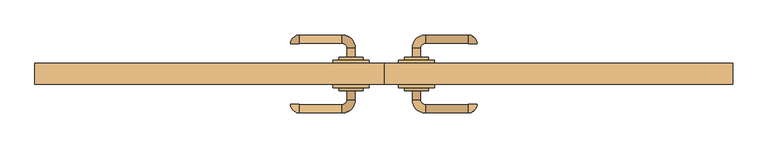
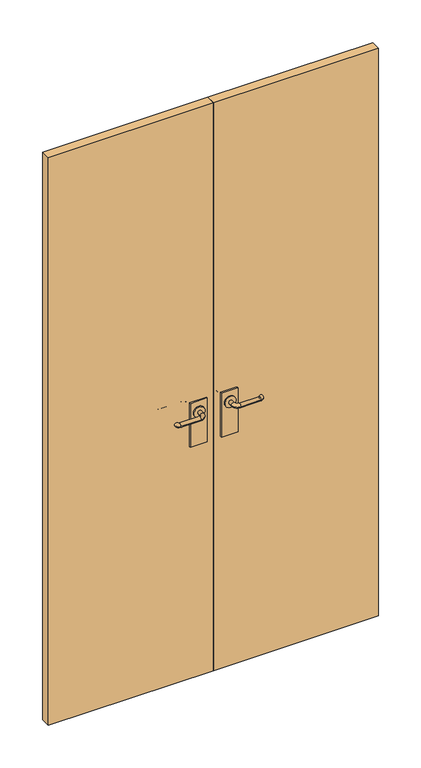
"""IFC4 building model written with IfcOpenShell, lengths in millimetres: door geometry, Porta Dupla de Abrir : 120x210cm - Marco Metálico."""

from ifc_helpers import new_model, si_unit, point, frame, frame_2d, origin, place, context, project, spatial, polyline, circle_curve, ellipse_curve, trimmed, segment, composite_curve, outline, extrude, source, transform, mapped, element, save
from ifc_brep_helpers import plane_surface, cylinder_surface, revolved_surface, advanced_brep


def door_43807c05(model_context):
    return source(origin(), model_context, "Body", "SolidModel", [
        extrude(outline(composite_curve([segment(trimmed(circle_curve(frame_2d((1050.0, -55.0)), 20.0), [point((1050.0, -35.0))], [point((1050.0, -75.0))], False, "CARTESIAN"), True, "CONTINUOUS"), segment(trimmed(circle_curve(frame_2d((1050.0, -55.0)), 20.0), [point((1050.0, -75.0))], [point((1050.0, -35.0))], False, "CARTESIAN"), True, "CONTINUOUS")], self_intersect=False)), frame((0.0, 50.0070105, 0.0), z_axis=(0.0, 1.0, 0.0), x_axis=(0.0, 0.0, 1.0)), (0.0, 0.0, 1.0), 4.5929895),
        advanced_brep(
        [(-62.0, 50.0070105, 1050.0), (-48.0, 50.0070105, 1050.0), (-62.0, 34.6, 1050.0), (-48.0, 34.6, 1050.0), (-70.0, 12.6, 1050.0), (-70.0, 26.6, 1050.0), (-142.0, 26.6, 1050.0), (-142.0, 12.6, 1050.0), (-143.0, 27.6, 1050.0), (-157.0, 27.6, 1050.0)],
        [
            (0, 1, circle_curve(frame((-55.0, 50.0070105, 1050.0), z_axis=(0.0, 1.0, 0.0), x_axis=(1.0, 0.0, 0.0)), 7.0)),
            (1, 0, circle_curve(frame((-55.0, 50.0070105, 1050.0), z_axis=(0.0, 1.0, 0.0), x_axis=(1.0, 0.0, 0.0)), 7.0)),
            (0, 2),
            (2, 3, circle_curve(frame((-55.0, 34.6, 1050.0), z_axis=(0.0, 1.0, 0.0), x_axis=(1.0, 0.0, 0.0)), 7.0)),
            (3, 1),
            (3, 2, circle_curve(frame((-55.0, 34.6, 1050.0), z_axis=(0.0, 1.0, 0.0), x_axis=(1.0, 0.0, 0.0)), 7.0)),
            (4, 3, circle_curve(frame((-70.0, 34.6, 1050.0), z_axis=(0.0, 0.0, 1.0), x_axis=(1.0, 0.0, 0.0)), 22.0)),
            (2, 5, circle_curve(frame((-70.0, 34.6, 1050.0), z_axis=(0.0, 0.0, -1.0), x_axis=(1.0, 0.0, 0.0)), 8.0)),
            (5, 4, circle_curve(frame((-70.0, 19.6, 1050.0), z_axis=(1.0, 0.0, 0.0), x_axis=(0.0, -1.0, 0.0)), 7.0)),
            (4, 5, circle_curve(frame((-70.0, 19.6, 1050.0), z_axis=(1.0, 0.0, 0.0), x_axis=(0.0, -1.0, 0.0)), 7.0)),
            (5, 6),
            (6, 7, circle_curve(frame((-142.0, 19.6, 1050.0), z_axis=(1.0, 0.0, 0.0), x_axis=(0.0, -1.0, 0.0)), 7.0)),
            (7, 4),
            (7, 6, circle_curve(frame((-142.0, 19.6, 1050.0), z_axis=(1.0, 0.0, 0.0), x_axis=(0.0, -1.0, 0.0)), 7.0)),
            (8, 9, circle_curve(frame((-150.0, 27.6, 1050.0), z_axis=(0.0, 1.0, 0.0), x_axis=(-1.0, 0.0, 0.0)), 7.0)),
            (9, 8, circle_curve(frame((-150.0, 27.6, 1050.0), z_axis=(0.0, 1.0, 0.0), x_axis=(-1.0, 0.0, 0.0)), 7.0)),
            (9, 7, circle_curve(frame((-142.0, 27.6, 1050.0), z_axis=(0.0, 0.0, 1.0), x_axis=(0.0, -1.0, 0.0)), 15.0)),
            (6, 8, circle_curve(frame((-142.0, 27.6, 1050.0), z_axis=(0.0, 0.0, -1.0), x_axis=(0.0, -1.0, 0.0)), 1.0)),
        ],
        [
            plane_surface(frame((-55.0, 50.0070105, 1050.0), z_axis=(0.0, 1.0, 0.0), x_axis=(0.0, 0.0, 1.0))),
            cylinder_surface(frame((-55.0, 50.0070105, 1050.0), z_axis=(0.0, 1.0, 0.0), x_axis=(1.0, 0.0, 0.0)), 7.0),
            revolved_surface(trimmed(ellipse_curve(frame((-55.0, 34.6, 1050.0), z_axis=(0.0, 1.0, 0.0), x_axis=(1.0, 0.0, 0.0)), 7.0, 7.0), [point((-62.0, 34.6, 1050.0))], [point((-48.0, 34.6, 1050.0))], True, "CARTESIAN"), (-70.0, 34.6, 1050.0), (0.0, 0.0, -1.0)),
            revolved_surface(trimmed(ellipse_curve(frame((-55.0, 34.6, 1050.0), z_axis=(0.0, 1.0, 0.0), x_axis=(1.0, 0.0, 0.0)), 7.0, 7.0), [point((-48.0, 34.6, 1050.0))], [point((-62.0, 34.6, 1050.0))], True, "CARTESIAN"), (-70.0, 34.6, 1050.0), (0.0, 0.0, -1.0)),
            cylinder_surface(frame((-70.0, 19.6, 1050.0), z_axis=(1.0, 0.0, 0.0), x_axis=(0.0, -1.0, 0.0)), 7.0),
            plane_surface(frame((-150.0, 27.6, 1050.0), z_axis=(0.0, 1.0, 0.0), x_axis=(0.0, 0.0, 1.0))),
            revolved_surface(trimmed(ellipse_curve(frame((-142.0, 19.6, 1050.0), z_axis=(1.0, 0.0, 0.0), x_axis=(0.0, -1.0, 0.0)), 7.0, 7.0), [point((-142.0, 26.6, 1050.0))], [point((-142.0, 12.6, 1050.0))], True, "CARTESIAN"), (-142.0, 27.6, 1050.0), (0.0, 0.0, -1.0)),
            revolved_surface(trimmed(ellipse_curve(frame((-142.0, 19.6, 1050.0), z_axis=(1.0, 0.0, 0.0), x_axis=(0.0, -1.0, 0.0)), 7.0, 7.0), [point((-142.0, 12.6, 1050.0))], [point((-142.0, 26.6, 1050.0))], True, "CARTESIAN"), (-142.0, 27.6, 1050.0), (0.0, 0.0, -1.0)),
        ],
        [
            (0, [[1, 2]]),
            (1, [[-1, 3, 4, 5]]),
            (1, [[-2, -5, 6, -3]]),
            (2, [[7, -4, 8, 9]]),
            (3, [[-8, -6, -7, 10]]),
            (4, [[-9, 11, 12, 13]]),
            (4, [[-10, -13, 14, -11]]),
            (5, [[15, 16]]),
            (6, [[17, -12, 18, -16]]),
            (7, [[-18, -14, -17, -15]]),
        ],
    ),
        extrude(outline(polyline([(-85.0, 60.6), (-25.0, 60.6), (-25.0, 54.6), (-85.0, 54.6), (-85.0, 60.6)])), frame((0.0, 0.0, 925.0), z_axis=(0.0, 0.0, 1.0), x_axis=(1.0, 0.0, 0.0)), (0.0, 0.0, 1.0), 165.0),
        extrude(outline(composite_curve([segment(trimmed(circle_curve(frame_2d((1050.0, -55.0)), 20.0), [point((1050.0, -35.0))], [point((1050.0, -75.0))], False, "CARTESIAN"), True, "CONTINUOUS"), segment(trimmed(circle_curve(frame_2d((1050.0, -55.0)), 20.0), [point((1050.0, -75.0))], [point((1050.0, -35.0))], False, "CARTESIAN"), True, "CONTINUOUS")], self_intersect=False)), frame((0.0, 101.6, 0.0), z_axis=(0.0, 1.0, 0.0), x_axis=(0.0, 0.0, 1.0)), (0.0, 0.0, 1.0), 4.5929895),
        advanced_brep(
        [(-62.0, 106.1929895, 1050.0), (-48.0, 106.1929895, 1050.0), (-48.0, 121.6, 1050.0), (-62.0, 121.6, 1050.0), (-70.0, 143.6, 1050.0), (-70.0, 129.6, 1050.0), (-142.0, 143.6, 1050.0), (-142.0, 129.6, 1050.0), (-143.0, 128.6, 1050.0), (-157.0, 128.6, 1050.0)],
        [
            (0, 1, circle_curve(frame((-55.0, 106.1929895, 1050.0), z_axis=(0.0, -1.0, 0.0), x_axis=(1.0, 0.0, 0.0)), 7.0)),
            (1, 0, circle_curve(frame((-55.0, 106.1929895, 1050.0), z_axis=(0.0, -1.0, 0.0), x_axis=(1.0, 0.0, 0.0)), 7.0)),
            (1, 2),
            (2, 3, circle_curve(frame((-55.0, 121.6, 1050.0), z_axis=(0.0, -1.0, 0.0), x_axis=(1.0, 0.0, 0.0)), 7.0)),
            (3, 0),
            (3, 2, circle_curve(frame((-55.0, 121.6, 1050.0), z_axis=(0.0, -1.0, 0.0), x_axis=(1.0, 0.0, 0.0)), 7.0)),
            (4, 5, circle_curve(frame((-70.0, 136.6, 1050.0), z_axis=(1.0, 0.0, 0.0), x_axis=(0.0, 1.0, 0.0)), 7.0)),
            (5, 3, circle_curve(frame((-70.0, 121.6, 1050.0), z_axis=(0.0, 0.0, -1.0), x_axis=(1.0, 0.0, 0.0)), 8.0)),
            (2, 4, circle_curve(frame((-70.0, 121.6, 1050.0), z_axis=(0.0, 0.0, 1.0), x_axis=(1.0, 0.0, 0.0)), 22.0)),
            (5, 4, circle_curve(frame((-70.0, 136.6, 1050.0), z_axis=(1.0, 0.0, 0.0), x_axis=(0.0, 1.0, 0.0)), 7.0)),
            (4, 6),
            (6, 7, circle_curve(frame((-142.0, 136.6, 1050.0), z_axis=(1.0, 0.0, 0.0), x_axis=(0.0, 1.0, 0.0)), 7.0)),
            (7, 5),
            (7, 6, circle_curve(frame((-142.0, 136.6, 1050.0), z_axis=(1.0, 0.0, 0.0), x_axis=(0.0, 1.0, 0.0)), 7.0)),
            (8, 9, circle_curve(frame((-150.0, 128.6, 1050.0), z_axis=(0.0, -1.0, 0.0), x_axis=(-1.0, 0.0, 0.0)), 7.0)),
            (9, 8, circle_curve(frame((-150.0, 128.6, 1050.0), z_axis=(0.0, -1.0, 0.0), x_axis=(-1.0, 0.0, 0.0)), 7.0)),
            (8, 7, circle_curve(frame((-142.0, 128.6, 1050.0), z_axis=(0.0, 0.0, -1.0), x_axis=(0.0, 1.0, 0.0)), 1.0)),
            (6, 9, circle_curve(frame((-142.0, 128.6, 1050.0), z_axis=(0.0, 0.0, 1.0), x_axis=(0.0, 1.0, 0.0)), 15.0)),
        ],
        [
            plane_surface(frame((-55.0, 106.1929895, 1050.0), z_axis=(0.0, -1.0, 0.0), x_axis=(0.0, 0.0, 1.0))),
            cylinder_surface(frame((-55.0, 106.1929895, 1050.0), z_axis=(0.0, -1.0, 0.0), x_axis=(1.0, 0.0, 0.0)), 7.0),
            revolved_surface(trimmed(ellipse_curve(frame((-55.0, 121.6, 1050.0), z_axis=(0.0, 1.0, 0.0), x_axis=(1.0, 0.0, 0.0)), 7.0, 7.0), [point((-62.0, 121.6, 1050.0))], [point((-48.0, 121.6, 1050.0))], True, "CARTESIAN"), (-70.0, 121.6, 1050.0), (0.0, 0.0, -1.0)),
            revolved_surface(trimmed(ellipse_curve(frame((-55.0, 121.6, 1050.0), z_axis=(0.0, 1.0, 0.0), x_axis=(1.0, 0.0, 0.0)), 7.0, 7.0), [point((-48.0, 121.6, 1050.0))], [point((-62.0, 121.6, 1050.0))], True, "CARTESIAN"), (-70.0, 121.6, 1050.0), (0.0, 0.0, -1.0)),
            cylinder_surface(frame((-70.0, 136.6, 1050.0), z_axis=(1.0, 0.0, 0.0), x_axis=(0.0, 1.0, 0.0)), 7.0),
            plane_surface(frame((-150.0, 128.6, 1050.0), z_axis=(0.0, -1.0, 0.0), x_axis=(0.0, 0.0, 1.0))),
            revolved_surface(trimmed(ellipse_curve(frame((-142.0, 136.6, 1050.0), z_axis=(-1.0, 0.0, 0.0), x_axis=(0.0, 1.0, 0.0)), 7.0, 7.0), [point((-142.0, 129.6, 1050.0))], [point((-142.0, 143.6, 1050.0))], True, "CARTESIAN"), (-142.0, 128.6, 1050.0), (0.0, 0.0, -1.0)),
            revolved_surface(trimmed(ellipse_curve(frame((-142.0, 136.6, 1050.0), z_axis=(-1.0, 0.0, 0.0), x_axis=(0.0, 1.0, 0.0)), 7.0, 7.0), [point((-142.0, 143.6, 1050.0))], [point((-142.0, 129.6, 1050.0))], True, "CARTESIAN"), (-142.0, 128.6, 1050.0), (0.0, 0.0, -1.0)),
        ],
        [
            (0, [[1, 2]]),
            (1, [[3, 4, 5, -2]]),
            (1, [[-5, 6, -3, -1]]),
            (2, [[7, 8, -4, 9]]),
            (3, [[10, -9, -6, -8]]),
            (4, [[11, 12, 13, -7]]),
            (4, [[-13, 14, -11, -10]]),
            (5, [[15, 16]]),
            (6, [[-15, 17, -12, 18]]),
            (7, [[-16, -18, -14, -17]]),
        ],
    ),
        extrude(outline(polyline([(-85.0, 95.6), (-85.0, 101.6), (-25.0, 101.6), (-25.0, 95.6), (-85.0, 95.6)])), frame((0.0, 0.0, 925.0), z_axis=(0.0, 0.0, 1.0), x_axis=(1.0, 0.0, 0.0)), (0.0, 0.0, 1.0), 165.0),
        extrude(outline(composite_curve([segment(trimmed(circle_curve(frame_2d((1050.0, 55.0)), 20.0), [point((1050.0, 35.0))], [point((1050.0, 75.0))], False, "CARTESIAN"), True, "CONTINUOUS"), segment(trimmed(circle_curve(frame_2d((1050.0, 55.0)), 20.0), [point((1050.0, 75.0))], [point((1050.0, 35.0))], False, "CARTESIAN"), True, "CONTINUOUS")], self_intersect=False)), frame((0.0, 50.0070105, 0.0), z_axis=(0.0, 1.0, 0.0), x_axis=(0.0, 0.0, 1.0)), (0.0, 0.0, 1.0), 4.5929895),
        advanced_brep(
        [(62.0, 50.0070105, 1050.0), (48.0, 50.0070105, 1050.0), (48.0, 34.6, 1050.0), (62.0, 34.6, 1050.0), (70.0, 12.6, 1050.0), (70.0, 26.6, 1050.0), (142.0, 12.6, 1050.0), (142.0, 26.6, 1050.0), (143.0, 27.6, 1050.0), (157.0, 27.6, 1050.0)],
        [
            (0, 1, circle_curve(frame((55.0, 50.0070105, 1050.0), z_axis=(0.0, 1.0, 0.0), x_axis=(-1.0, 0.0, 0.0)), 7.0)),
            (1, 0, circle_curve(frame((55.0, 50.0070105, 1050.0), z_axis=(0.0, 1.0, 0.0), x_axis=(-1.0, 0.0, 0.0)), 7.0)),
            (1, 2),
            (2, 3, circle_curve(frame((55.0, 34.6, 1050.0), z_axis=(0.0, 1.0, 0.0), x_axis=(-1.0, 0.0, 0.0)), 7.0)),
            (3, 0),
            (3, 2, circle_curve(frame((55.0, 34.6, 1050.0), z_axis=(0.0, 1.0, 0.0), x_axis=(-1.0, 0.0, 0.0)), 7.0)),
            (4, 5, circle_curve(frame((70.0, 19.6, 1050.0), z_axis=(-1.0, 0.0, 0.0), x_axis=(0.0, -1.0, 0.0)), 7.0)),
            (5, 3, circle_curve(frame((70.0, 34.6, 1050.0), z_axis=(0.0, 0.0, -1.0), x_axis=(-1.0, 0.0, 0.0)), 8.0)),
            (2, 4, circle_curve(frame((70.0, 34.6, 1050.0), z_axis=(0.0, 0.0, 1.0), x_axis=(-1.0, 0.0, 0.0)), 22.0)),
            (5, 4, circle_curve(frame((70.0, 19.6, 1050.0), z_axis=(-1.0, 0.0, 0.0), x_axis=(0.0, -1.0, 0.0)), 7.0)),
            (4, 6),
            (6, 7, circle_curve(frame((142.0, 19.6, 1050.0), z_axis=(-1.0, 0.0, 0.0), x_axis=(0.0, -1.0, 0.0)), 7.0)),
            (7, 5),
            (7, 6, circle_curve(frame((142.0, 19.6, 1050.0), z_axis=(-1.0, 0.0, 0.0), x_axis=(0.0, -1.0, 0.0)), 7.0)),
            (8, 9, circle_curve(frame((150.0, 27.6, 1050.0), z_axis=(0.0, 1.0, 0.0), x_axis=(1.0, 0.0, 0.0)), 7.0)),
            (9, 8, circle_curve(frame((150.0, 27.6, 1050.0), z_axis=(0.0, 1.0, 0.0), x_axis=(1.0, 0.0, 0.0)), 7.0)),
            (8, 7, circle_curve(frame((142.0, 27.6, 1050.0), z_axis=(0.0, 0.0, -1.0), x_axis=(0.0, -1.0, 0.0)), 1.0)),
            (6, 9, circle_curve(frame((142.0, 27.6, 1050.0), z_axis=(0.0, 0.0, 1.0), x_axis=(0.0, -1.0, 0.0)), 15.0)),
        ],
        [
            plane_surface(frame((55.0, 50.0070105, 1050.0), z_axis=(0.0, 1.0, 0.0), x_axis=(0.0, 0.0, 1.0))),
            cylinder_surface(frame((55.0, 50.0070105, 1050.0), z_axis=(0.0, 1.0, 0.0), x_axis=(-1.0, 0.0, 0.0)), 7.0),
            revolved_surface(trimmed(ellipse_curve(frame((55.0, 34.6, 1050.0), z_axis=(0.0, -1.0, 0.0), x_axis=(-1.0, 0.0, 0.0)), 7.0, 7.0), [point((62.0, 34.6, 1050.0))], [point((48.0, 34.6, 1050.0))], True, "CARTESIAN"), (70.0, 34.6, 1050.0), (0.0, 0.0, -1.0)),
            revolved_surface(trimmed(ellipse_curve(frame((55.0, 34.6, 1050.0), z_axis=(0.0, -1.0, 0.0), x_axis=(-1.0, 0.0, 0.0)), 7.0, 7.0), [point((48.0, 34.6, 1050.0))], [point((62.0, 34.6, 1050.0))], True, "CARTESIAN"), (70.0, 34.6, 1050.0), (0.0, 0.0, -1.0)),
            cylinder_surface(frame((70.0, 19.6, 1050.0), z_axis=(-1.0, 0.0, 0.0), x_axis=(0.0, -1.0, 0.0)), 7.0),
            plane_surface(frame((150.0, 27.6, 1050.0), z_axis=(0.0, 1.0, 0.0), x_axis=(0.0, 0.0, 1.0))),
            revolved_surface(trimmed(ellipse_curve(frame((142.0, 19.6, 1050.0), z_axis=(1.0, 0.0, 0.0), x_axis=(0.0, -1.0, 0.0)), 7.0, 7.0), [point((142.0, 26.6, 1050.0))], [point((142.0, 12.6, 1050.0))], True, "CARTESIAN"), (142.0, 27.6, 1050.0), (0.0, 0.0, -1.0)),
            revolved_surface(trimmed(ellipse_curve(frame((142.0, 19.6, 1050.0), z_axis=(1.0, 0.0, 0.0), x_axis=(0.0, -1.0, 0.0)), 7.0, 7.0), [point((142.0, 12.6, 1050.0))], [point((142.0, 26.6, 1050.0))], True, "CARTESIAN"), (142.0, 27.6, 1050.0), (0.0, 0.0, -1.0)),
        ],
        [
            (0, [[1, 2]]),
            (1, [[3, 4, 5, -2]]),
            (1, [[-5, 6, -3, -1]]),
            (2, [[7, 8, -4, 9]]),
            (3, [[10, -9, -6, -8]]),
            (4, [[11, 12, 13, -7]]),
            (4, [[-13, 14, -11, -10]]),
            (5, [[15, 16]]),
            (6, [[-15, 17, -12, 18]]),
            (7, [[-16, -18, -14, -17]]),
        ],
    ),
        extrude(outline(polyline([(85.0, 60.6), (85.0, 54.6), (25.0, 54.6), (25.0, 60.6), (85.0, 60.6)])), frame((0.0, 0.0, 925.0), z_axis=(0.0, 0.0, 1.0), x_axis=(1.0, 0.0, 0.0)), (0.0, 0.0, 1.0), 165.0),
        extrude(outline(composite_curve([segment(trimmed(circle_curve(frame_2d((1050.0, 55.0)), 20.0), [point((1050.0, 35.0))], [point((1050.0, 75.0))], False, "CARTESIAN"), True, "CONTINUOUS"), segment(trimmed(circle_curve(frame_2d((1050.0, 55.0)), 20.0), [point((1050.0, 75.0))], [point((1050.0, 35.0))], False, "CARTESIAN"), True, "CONTINUOUS")], self_intersect=False)), frame((0.0, 101.6, 0.0), z_axis=(0.0, 1.0, 0.0), x_axis=(0.0, 0.0, 1.0)), (0.0, 0.0, 1.0), 4.5929895),
        advanced_brep(
        [(62.0, 106.1929895, 1050.0), (48.0, 106.1929895, 1050.0), (62.0, 121.6, 1050.0), (48.0, 121.6, 1050.0), (70.0, 143.6, 1050.0), (70.0, 129.6, 1050.0), (142.0, 129.6, 1050.0), (142.0, 143.6, 1050.0), (143.0, 128.6, 1050.0), (157.0, 128.6, 1050.0)],
        [
            (0, 1, circle_curve(frame((55.0, 106.1929895, 1050.0), z_axis=(0.0, -1.0, 0.0), x_axis=(-1.0, 0.0, 0.0)), 7.0)),
            (1, 0, circle_curve(frame((55.0, 106.1929895, 1050.0), z_axis=(0.0, -1.0, 0.0), x_axis=(-1.0, 0.0, 0.0)), 7.0)),
            (0, 2),
            (2, 3, circle_curve(frame((55.0, 121.6, 1050.0), z_axis=(0.0, -1.0, 0.0), x_axis=(-1.0, 0.0, 0.0)), 7.0)),
            (3, 1),
            (3, 2, circle_curve(frame((55.0, 121.6, 1050.0), z_axis=(0.0, -1.0, 0.0), x_axis=(-1.0, 0.0, 0.0)), 7.0)),
            (4, 3, circle_curve(frame((70.0, 121.6, 1050.0), z_axis=(0.0, 0.0, 1.0), x_axis=(-1.0, 0.0, 0.0)), 22.0)),
            (2, 5, circle_curve(frame((70.0, 121.6, 1050.0), z_axis=(0.0, 0.0, -1.0), x_axis=(-1.0, 0.0, 0.0)), 8.0)),
            (5, 4, circle_curve(frame((70.0, 136.6, 1050.0), z_axis=(-1.0, 0.0, 0.0), x_axis=(0.0, 1.0, 0.0)), 7.0)),
            (4, 5, circle_curve(frame((70.0, 136.6, 1050.0), z_axis=(-1.0, 0.0, 0.0), x_axis=(0.0, 1.0, 0.0)), 7.0)),
            (5, 6),
            (6, 7, circle_curve(frame((142.0, 136.6, 1050.0), z_axis=(-1.0, 0.0, 0.0), x_axis=(0.0, 1.0, 0.0)), 7.0)),
            (7, 4),
            (7, 6, circle_curve(frame((142.0, 136.6, 1050.0), z_axis=(-1.0, 0.0, 0.0), x_axis=(0.0, 1.0, 0.0)), 7.0)),
            (8, 9, circle_curve(frame((150.0, 128.6, 1050.0), z_axis=(0.0, -1.0, 0.0), x_axis=(1.0, 0.0, 0.0)), 7.0)),
            (9, 8, circle_curve(frame((150.0, 128.6, 1050.0), z_axis=(0.0, -1.0, 0.0), x_axis=(1.0, 0.0, 0.0)), 7.0)),
            (9, 7, circle_curve(frame((142.0, 128.6, 1050.0), z_axis=(0.0, 0.0, 1.0), x_axis=(0.0, 1.0, 0.0)), 15.0)),
            (6, 8, circle_curve(frame((142.0, 128.6, 1050.0), z_axis=(0.0, 0.0, -1.0), x_axis=(0.0, 1.0, 0.0)), 1.0)),
        ],
        [
            plane_surface(frame((55.0, 106.1929895, 1050.0), z_axis=(0.0, -1.0, 0.0), x_axis=(0.0, 0.0, 1.0))),
            cylinder_surface(frame((55.0, 106.1929895, 1050.0), z_axis=(0.0, -1.0, 0.0), x_axis=(-1.0, 0.0, 0.0)), 7.0),
            revolved_surface(trimmed(ellipse_curve(frame((55.0, 121.6, 1050.0), z_axis=(0.0, -1.0, 0.0), x_axis=(-1.0, 0.0, 0.0)), 7.0, 7.0), [point((62.0, 121.6, 1050.0))], [point((48.0, 121.6, 1050.0))], True, "CARTESIAN"), (70.0, 121.6, 1050.0), (0.0, 0.0, -1.0)),
            revolved_surface(trimmed(ellipse_curve(frame((55.0, 121.6, 1050.0), z_axis=(0.0, -1.0, 0.0), x_axis=(-1.0, 0.0, 0.0)), 7.0, 7.0), [point((48.0, 121.6, 1050.0))], [point((62.0, 121.6, 1050.0))], True, "CARTESIAN"), (70.0, 121.6, 1050.0), (0.0, 0.0, -1.0)),
            cylinder_surface(frame((70.0, 136.6, 1050.0), z_axis=(-1.0, 0.0, 0.0), x_axis=(0.0, 1.0, 0.0)), 7.0),
            plane_surface(frame((150.0, 128.6, 1050.0), z_axis=(0.0, -1.0, 0.0), x_axis=(0.0, 0.0, 1.0))),
            revolved_surface(trimmed(ellipse_curve(frame((142.0, 136.6, 1050.0), z_axis=(-1.0, 0.0, 0.0), x_axis=(0.0, 1.0, 0.0)), 7.0, 7.0), [point((142.0, 129.6, 1050.0))], [point((142.0, 143.6, 1050.0))], True, "CARTESIAN"), (142.0, 128.6, 1050.0), (0.0, 0.0, -1.0)),
            revolved_surface(trimmed(ellipse_curve(frame((142.0, 136.6, 1050.0), z_axis=(-1.0, 0.0, 0.0), x_axis=(0.0, 1.0, 0.0)), 7.0, 7.0), [point((142.0, 143.6, 1050.0))], [point((142.0, 129.6, 1050.0))], True, "CARTESIAN"), (142.0, 128.6, 1050.0), (0.0, 0.0, -1.0)),
        ],
        [
            (0, [[1, 2]]),
            (1, [[-1, 3, 4, 5]]),
            (1, [[-2, -5, 6, -3]]),
            (2, [[7, -4, 8, 9]]),
            (3, [[-8, -6, -7, 10]]),
            (4, [[-9, 11, 12, 13]]),
            (4, [[-10, -13, 14, -11]]),
            (5, [[15, 16]]),
            (6, [[17, -12, 18, -16]]),
            (7, [[-18, -14, -17, -15]]),
        ],
    ),
        extrude(outline(polyline([(85.0, 95.6), (25.0, 95.6), (25.0, 101.6), (85.0, 101.6), (85.0, 95.6)])), frame((0.0, 0.0, 925.0), z_axis=(0.0, 0.0, 1.0), x_axis=(1.0, 0.0, 0.0)), (0.0, 0.0, 1.0), 165.0),
        extrude(outline(polyline([(0.0, 60.6), (-587.0, 60.6), (-587.0, 95.6), (0.0, 95.6), (0.0, 60.6)])), frame((0.0, 0.0, 53.0), z_axis=(0.0, 0.0, 1.0), x_axis=(1.0, 0.0, 0.0)), (0.0, 0.0, 1.0), 2133.0),
        extrude(outline(polyline([(587.0, 60.6), (0.0, 60.6), (0.0, 95.6), (587.0, 95.6), (587.0, 60.6)])), frame((0.0, 0.0, 53.0), z_axis=(0.0, 0.0, 1.0), x_axis=(1.0, 0.0, 0.0)), (0.0, 0.0, 1.0), 2133.0),
    ])


if __name__ == "__main__":
    model = new_model("IFC4")
    model_context = context("Model", 3, world=origin())
    ifc_project = project(units=[si_unit("LENGTHUNIT", "METRE", prefix="MILLI")], contexts=[model_context])
    site = spatial("IfcSite", under=ifc_project)
    building = spatial("IfcBuilding", under=site)
    placement = place(None, origin())
    door_shape = door_43807c05(model_context)
    element("IfcDoor", 1, ObjectType="Porta Dupla de Abrir : 120x210cm - Marco Metálico", at=placement, inside=building, context=model_context, shape_type="MappedRepresentation", body=[
        mapped(door_shape, transform((0.0, 0.0, 0.0), x_axis=(1.0, 0.0, 0.0), y_axis=(0.0, 1.0, 0.0), z_axis=(0.0, 0.0, 1.0))),
    ])
    save(model, "model.ifc")

# Revit data of these elements
# Type "Porta Dupla de Abrir : 120x210cm - Marco Metálico"
#   Type Mark = ""
#   SINAPI = ""
#   Maçaneta [instance default] = ""
#   Fechadura [instance default] = ""
#   Vão Luz (somente para informação) = 114.80 cm
#   Tolerância Folha Vertical = 0.30 cm
#   Módulo Básico M = 10.00 cm
#   Largura de Coordenação Modular Largura CM = 120.00 cm
#   Rough Width = 120.00 cm
#   Deslocamento da Horizontal da Folha = 1.00 cm
#   Altura de Coordenação Modular Largura CM = 220.00 cm
#   Rough Height = 220.00 cm
#   Altura Nominal = 212.40 cm
#   Ajuste de Coordenação Topo AC Topo = 0.00 cm
#   Ajuste de Coordenação Base AC Base = 5.00 cm
#   Ajuste de Coordenação AC = 0.00 cm
#   Tolerância Folha Horizontal = 0.20 cm
#   Largura Folha (somente para informação) = 58.70 cm
#   Espessura Folha = 3.50 cm
#   Maçaneta - Distância da Folha = 5.50 cm
#   Maçaneta - Altura = 100.00 cm
#   Largura Nominal (Largura Mn) = 117.80 cm
#   Distância do Nível = 0.30 cm
#   Aduela Interna Espessura = 1.10 cm
#   Aduela Externa Espessura = 2.60 cm
#   Altura Folha (somente para informação) = 211.90 cm
#   Height = 215.00 cm
#   Width = 120.00 cm
#   Número de Módulos Básicos nM Largura = 12
#   Número de Módulos Básicos nM Altura = 22
#   Marco Metálico = yes
#   Aduela de Madeira = no
#   Aduela Metálica de Canto = no
#   Guarnição Chanfrada = no
#   Batente - Material [instance default] = none
#   Painel - Material [instance default] = none
#   Construction Type = (empty or 0)
#   Model = ""
#   Function = (empty or 0)
#   Description = (empty or 0)
#   Wall Closure = (empty or 0)
#   Assembly Code = ""
# Element 1 (IfcDoor, "Porta Dupla de Abrir : 120x210cm - Marco Metálico")
#   Materials on its faces: "Porta - Maçaneta"
# Materials
#   "Porta - Maçaneta": class "Metal", colour RGB 189 187 185, transparency 0, Cost = 0
